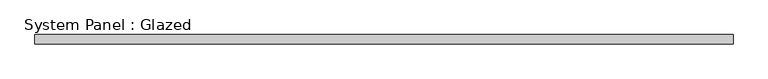
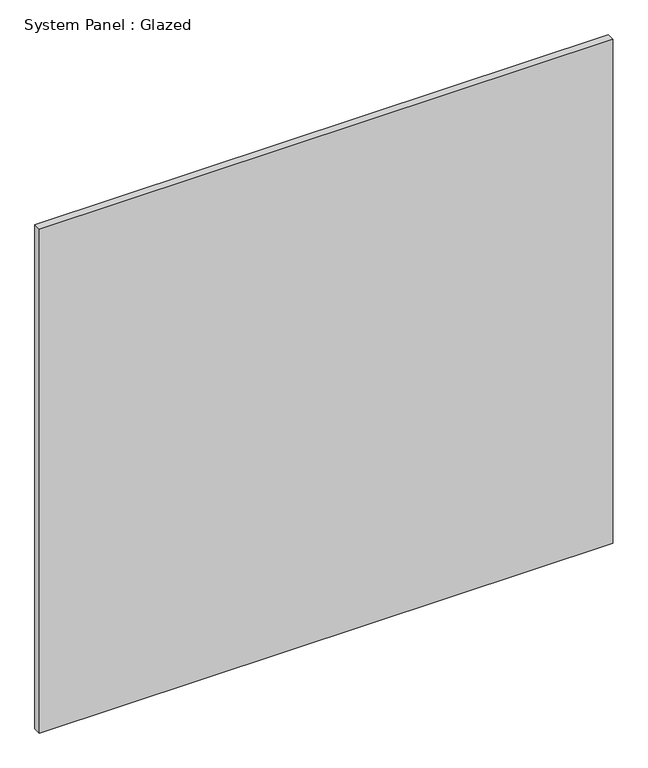
"""IFC4 building model written with IfcOpenShell, lengths in millimetres: plate geometry, System Panel : Glazed."""

from ifc_helpers import new_model, si_unit, origin, origin_with_axes, place, context, project, spatial, polyline, outline, extrude, source, transform, mapped, element, save


def system_panel_glazed_71f58c71(model_context):
    return source(origin(), model_context, "Body", "SweptSolid", [
        extrude(outline(polyline([(915.0000002, 24.5), (-915.0000002, 24.5), (-915.0000002, 49.5), (915.0000002, 49.5), (915.0000002, 24.5)])), origin_with_axes(), (0.0, 0.0, 1.0), 1699.4222628),
    ])


if __name__ == "__main__":
    model = new_model("IFC4")
    model_context = context("Model", 3, world=origin())
    ifc_project = project(units=[si_unit("LENGTHUNIT", "METRE", prefix="MILLI")], contexts=[model_context])
    site = spatial("IfcSite", under=ifc_project)
    building = spatial("IfcBuilding", under=site)
    placement = place(None, origin())
    system_panel_glazed_shape = system_panel_glazed_71f58c71(model_context)
    element("IfcPlate", 1, ObjectType="System Panel : Glazed", at=placement, inside=building, context=model_context, shape_type="MappedRepresentation", body=[
        mapped(system_panel_glazed_shape, transform((0.0, 0.0, 0.0), x_axis=(1.0, 0.0, 0.0), y_axis=(0.0, 1.0, 0.0), z_axis=(0.0, 0.0, 1.0))),
    ])
    save(model, "model.ifc")

# Revit data of these elements
# Element 1 (IfcPlate, "System Panel : Glazed")
#   Materials on its faces: "Glass"
# Materials
#   "Glass": class "Glass", colour RGB 218 227 224, transparency 0.85, Description = "Soda Lime Glass", Cost = 0
